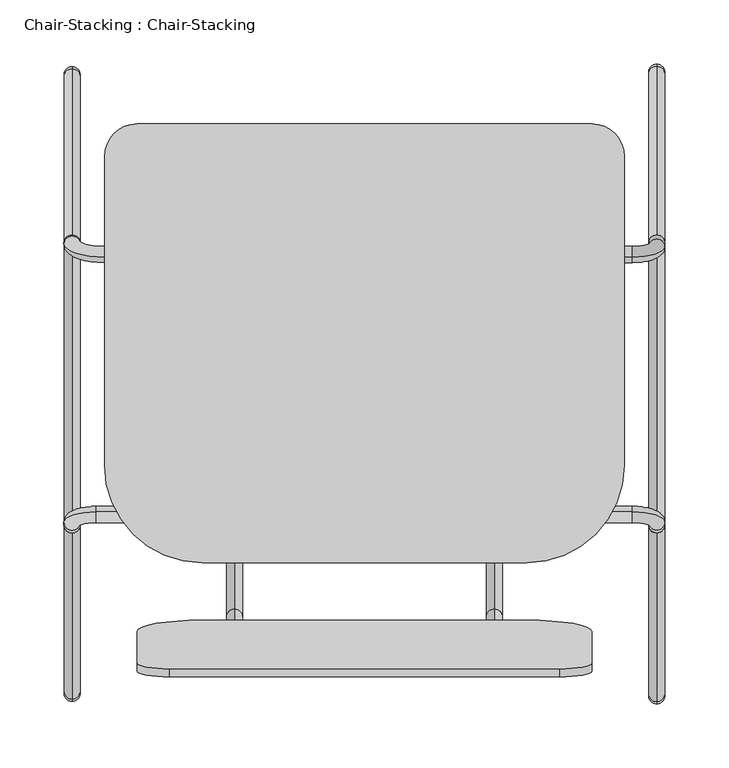
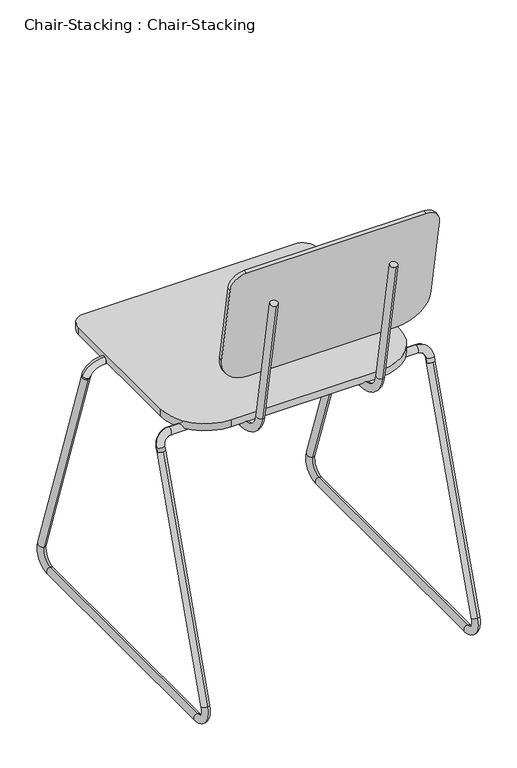
"""IFC4 building model written with IfcOpenShell, lengths in millimetres: furniture geometry, Chair-Stacking : Chair-Stacking."""

from ifc_helpers import new_model, si_unit, point, frame, frame_2d, origin, place, context, project, spatial, polyline, circle_curve, ellipse_curve, trimmed, segment, composite_curve, outline, extrude, source, transform, mapped, element, save
from ifc_brep_helpers import plane_surface, cylinder_surface, revolved_surface, advanced_brep


def chair_stacking_chair_stacking_76f41a28(model_context):
    return source(origin(), model_context, "Body", "SolidModel", [
        advanced_brep(
        [(-280.6491803, 213.2656675, 431.8), (-280.6491803, 213.2656675, 444.5), (-280.6491803, -23.0277124, 431.8), (-280.6491803, -23.0277124, 444.5), (-280.6491803, -66.802417, 481.2313385), (-280.6491803, -79.3094755, 479.0260066), (-280.6491803, -119.2282049, 705.4163709), (-280.6491803, -106.7211464, 707.6217027)],
        [
            (0, 1, circle_curve(frame((-280.6491803, 213.2656675, 438.15), z_axis=(0.0, 1.0, 0.0), x_axis=(0.0, 0.0, 1.0)), 6.35)),
            (1, 0, circle_curve(frame((-280.6491803, 213.2656675, 438.15), z_axis=(0.0, 1.0, 0.0), x_axis=(0.0, 0.0, 1.0)), 6.35)),
            (0, 2),
            (2, 3, circle_curve(frame((-280.6491803, -23.0277124, 438.15), z_axis=(0.0, 1.0, 0.0), x_axis=(0.0, 0.0, 1.0)), 6.35)),
            (3, 1),
            (3, 2, circle_curve(frame((-280.6491803, -23.0277124, 438.15), z_axis=(0.0, 1.0, 0.0), x_axis=(0.0, 0.0, 1.0)), 6.35)),
            (4, 3, circle_curve(frame((-280.6491803, -23.0277124, 488.95), z_axis=(1.0, 0.0, 0.0), x_axis=(0.0, 0.0, -1.0)), 44.45)),
            (2, 5, circle_curve(frame((-280.6491803, -23.0277124, 488.95), z_axis=(-1.0, 0.0, 0.0), x_axis=(0.0, 0.0, -1.0)), 57.15)),
            (5, 4, circle_curve(frame((-280.6491803, -73.0559463, 480.1286726), z_axis=(0.0, 0.17364817766693444, -0.9848077530122074), x_axis=(0.0, 0.9848077530122074, 0.17364817766693444)), 6.35)),
            (4, 5, circle_curve(frame((-280.6491803, -73.0559463, 480.1286726), z_axis=(0.0, 0.17364817766693444, -0.9848077530122074), x_axis=(0.0, 0.9848077530122074, 0.17364817766693444)), 6.35)),
            (6, 7, circle_curve(frame((-280.6491803, -112.9746757, 706.5190368), z_axis=(0.0, -0.1736481776669348, 0.9848077530122074), x_axis=(0.0, 0.9848077530122074, 0.1736481776669348)), 6.35)),
            (7, 6, circle_curve(frame((-280.6491803, -112.9746757, 706.5190368), z_axis=(0.0, -0.1736481776669348, 0.9848077530122074), x_axis=(0.0, 0.9848077530122074, 0.1736481776669348)), 6.35)),
            (5, 6),
            (7, 4),
        ],
        [
            plane_surface(frame((-286.9991803, 213.2656675, 438.15), z_axis=(0.0, 1.0, 0.0), x_axis=(0.0, 0.0, -1.0))),
            cylinder_surface(frame((-280.6491803, 213.2656675, 438.15), z_axis=(0.0, 1.0, 0.0), x_axis=(0.0, 0.0, 1.0)), 6.35),
            revolved_surface(trimmed(ellipse_curve(frame((-280.6491803, -23.0277124, 438.15), z_axis=(0.0, 1.0, 0.0), x_axis=(0.0, 0.0, 1.0)), 6.35, 6.35), [point((-280.6491803, -23.0277124, 431.8))], [point((-280.6491803, -23.0277124, 444.5))], True, "CARTESIAN"), (-280.6491803, -23.0277124, 488.95), (-1.0, 0.0, 0.0)),
            revolved_surface(trimmed(ellipse_curve(frame((-280.6491803, -23.0277124, 438.15), z_axis=(0.0, 1.0, 0.0), x_axis=(0.0, 0.0, 1.0)), 6.35, 6.35), [point((-280.6491803, -23.0277124, 444.5))], [point((-280.6491803, -23.0277124, 431.8))], True, "CARTESIAN"), (-280.6491803, -23.0277124, 488.95), (-1.0, 0.0, 0.0)),
            plane_surface(frame((-280.6491803, -119.2282049, 705.4163709), z_axis=(0.0, -0.17364817766692842, 0.9848077530122085), x_axis=(1.0, 0.0, 0.0))),
            cylinder_surface(frame((-280.6491803, -73.0559463, 480.1286726), z_axis=(0.0, 0.1736481776669348, -0.9848077530122074), x_axis=(0.0, 0.9848077530122074, 0.1736481776669348)), 6.35),
        ],
        [
            (0, [[1, 2]]),
            (1, [[-1, 3, 4, 5]]),
            (1, [[-2, -5, 6, -3]]),
            (2, [[7, -4, 8, 9]]),
            (3, [[-8, -6, -7, 10]]),
            (4, [[11, 12]]),
            (5, [[-9, 13, -12, 14]]),
            (5, [[-10, -14, -11, -13]]),
        ],
    ),
        advanced_brep(
        [(-77.4491803, 213.2656675, 431.8), (-77.4491803, 213.2656675, 444.5), (-77.4491803, -23.0277124, 431.8), (-77.4491803, -23.0277124, 444.5), (-77.4491803, -66.802417, 481.2313385), (-77.4491803, -79.3094755, 479.0260066), (-77.4491803, -118.9339087, 703.7473341), (-77.4491803, -106.4268502, 705.9526659)],
        [
            (0, 1, circle_curve(frame((-77.4491803, 213.2656675, 438.15), z_axis=(0.0, 1.0, 0.0), x_axis=(0.0, 0.0, 1.0)), 6.35)),
            (1, 0, circle_curve(frame((-77.4491803, 213.2656675, 438.15), z_axis=(0.0, 1.0, 0.0), x_axis=(0.0, 0.0, 1.0)), 6.35)),
            (0, 2),
            (2, 3, circle_curve(frame((-77.4491803, -23.0277124, 438.15), z_axis=(0.0, 1.0, 0.0), x_axis=(0.0, 0.0, 1.0)), 6.35)),
            (3, 1),
            (3, 2, circle_curve(frame((-77.4491803, -23.0277124, 438.15), z_axis=(0.0, 1.0, 0.0), x_axis=(0.0, 0.0, 1.0)), 6.35)),
            (4, 3, circle_curve(frame((-77.4491803, -23.0277124, 488.95), z_axis=(1.0, 0.0, 0.0), x_axis=(0.0, 0.0, -1.0)), 44.45)),
            (2, 5, circle_curve(frame((-77.4491803, -23.0277124, 488.95), z_axis=(-1.0, 0.0, 0.0), x_axis=(0.0, 0.0, -1.0)), 57.15)),
            (5, 4, circle_curve(frame((-77.4491803, -73.0559463, 480.1286726), z_axis=(0.0, 0.1736481776669385, -0.9848077530122066), x_axis=(0.0, 0.9848077530122066, 0.1736481776669385)), 6.35)),
            (4, 5, circle_curve(frame((-77.4491803, -73.0559463, 480.1286726), z_axis=(0.0, 0.1736481776669372, -0.9848077530122068), x_axis=(0.0, 0.9848077530122068, 0.1736481776669372)), 6.35)),
            (6, 7, circle_curve(frame((-77.4491803, -112.6803794, 704.85), z_axis=(0.0, -0.17364817766693896, 0.9848077530122066), x_axis=(0.0, 0.9848077530122066, 0.17364817766693896)), 6.35)),
            (7, 6, circle_curve(frame((-77.4491803, -112.6803794, 704.85), z_axis=(0.0, -0.17364817766693896, 0.9848077530122066), x_axis=(0.0, 0.9848077530122066, 0.17364817766693896)), 6.35)),
            (5, 6),
            (7, 4),
        ],
        [
            plane_surface(frame((-83.7991803, 213.2656675, 438.15), z_axis=(0.0, 1.0, 0.0), x_axis=(0.0, 0.0, -1.0))),
            cylinder_surface(frame((-77.4491803, 213.2656675, 438.15), z_axis=(0.0, 1.0, 0.0), x_axis=(0.0, 0.0, 1.0)), 6.35),
            revolved_surface(trimmed(ellipse_curve(frame((-77.4491803, -23.0277124, 438.15), z_axis=(0.0, 1.0, 0.0), x_axis=(0.0, 0.0, 1.0)), 6.35, 6.35), [point((-77.4491803, -23.0277124, 431.8))], [point((-77.4491803, -23.0277124, 444.5))], True, "CARTESIAN"), (-77.4491803, -23.0277124, 488.95), (-1.0, 0.0, 0.0)),
            revolved_surface(trimmed(ellipse_curve(frame((-77.4491803, -23.0277124, 438.15), z_axis=(0.0, 1.0, 0.0), x_axis=(0.0, 0.0, 1.0)), 6.35, 6.35), [point((-77.4491803, -23.0277124, 444.5))], [point((-77.4491803, -23.0277124, 431.8))], True, "CARTESIAN"), (-77.4491803, -23.0277124, 488.95), (-1.0, 0.0, 0.0)),
            plane_surface(frame((-77.4491803, -118.9339087, 703.7473341), z_axis=(0.0, -0.17364817766692892, 0.9848077530122084), x_axis=(1.0, 0.0, 0.0))),
            cylinder_surface(frame((-77.4491803, -73.0559463, 480.1286726), z_axis=(0.0, 0.17364817766693896, -0.9848077530122066), x_axis=(0.0, 0.9848077530122066, 0.17364817766693896)), 6.35),
        ],
        [
            (0, [[1, 2]]),
            (1, [[-1, 3, 4, 5]]),
            (1, [[-2, -5, 6, -3]]),
            (2, [[7, -4, 8, 9]]),
            (3, [[-8, -6, -7, 10]]),
            (4, [[11, 12]]),
            (5, [[-9, 13, -12, 14]]),
            (5, [[-10, -14, -11, -13]]),
        ],
    ),
        extrude(outline(composite_curve([segment(trimmed(circle_curve(frame_2d((-1.2491803, 286.7314636)), 25.4), [point((-1.2491803, 312.1314636))], [point((24.1508197, 286.7314636))], False, "CARTESIAN"), True, "CONTINUOUS"), segment(polyline([(24.1508197, 286.7314636), (24.1508197, 45.4314636)]), True, "CONTINUOUS"), segment(trimmed(circle_curve(frame_2d((-52.0491803, 45.4314636)), 76.2), [point((24.1508197, 45.4314636))], [point((-52.0491803, -30.7685364))], False, "CARTESIAN"), True, "CONTINUOUS"), segment(polyline([(-52.0491803, -30.7685364), (-306.0491803, -30.7685364)]), True, "CONTINUOUS"), segment(trimmed(circle_curve(frame_2d((-306.0491803, 45.4314636)), 76.2), [point((-306.0491803, -30.7685364))], [point((-382.2491803, 45.4314636))], False, "CARTESIAN"), True, "CONTINUOUS"), segment(polyline([(-382.2491803, 45.4314636), (-382.2491803, 286.7314636)]), True, "CONTINUOUS"), segment(trimmed(circle_curve(frame_2d((-356.8491803, 286.7314636)), 25.4), [point((-382.2491803, 286.7314636))], [point((-356.8491803, 312.1314636))], False, "CARTESIAN"), True, "CONTINUOUS"), segment(polyline([(-356.8491803, 312.1314636), (-1.2491803, 312.1314636)]), True, "CONTINUOUS")], self_intersect=False)), frame((0.0, 0.0, 444.5), z_axis=(0.0, 0.0, 1.0), x_axis=(1.0, 0.0, 0.0)), (0.0, 0.0, 1.0), 12.7),
        extrude(outline(composite_curve([segment(polyline([(-304.8, 0.0), (0.0, 0.0)]), True, "CONTINUOUS"), segment(trimmed(circle_curve(frame_2d((0.0, -25.4)), 25.4), [point((0.0, 0.0))], [point((25.4, -25.4))], False, "CARTESIAN"), True, "CONTINUOUS"), segment(polyline([(25.4, -25.4), (25.4, -168.3013626)]), True, "CONTINUOUS"), segment(trimmed(circle_curve(frame_2d((-25.4, -168.3013626)), 50.8), [point((25.4, -168.3013626))], [point((-25.4, -219.1013626))], False, "CARTESIAN"), True, "CONTINUOUS"), segment(polyline([(-25.4, -219.1013626), (-279.4, -219.1013626)]), True, "CONTINUOUS"), segment(trimmed(circle_curve(frame_2d((-279.4, -168.3013626)), 50.8), [point((-279.4, -219.1013626))], [point((-330.2, -168.3013626))], False, "CARTESIAN"), True, "CONTINUOUS"), segment(polyline([(-330.2, -168.3013626), (-330.2, -25.4)]), True, "CONTINUOUS"), segment(trimmed(circle_curve(frame_2d((-304.8, -25.4)), 25.4), [point((-330.2, -25.4))], [point((-304.8, 0.0))], False, "CARTESIAN"), True, "CONTINUOUS")], self_intersect=False)), frame((-331.4491803, -119.9531376, 782.6640535), z_axis=(0.0, 0.9848077530122084, 0.17364817766692858), x_axis=(-1.0, 0.0, 0.0)), (0.0, 0.0, 1.0), 6.35),
        advanced_brep(
        [(55.9008197, 219.2327758, 419.1211728), (43.2008197, 219.2327758, 419.1211728), (55.9008197, 216.3017292, 427.6700586), (43.2008197, 216.3017292, 427.6700586), (30.5008197, 212.1828103, 439.6835721), (30.5008197, 208.0638914, 451.6970857), (-382.2491803, 208.0638914, 451.6970857), (-382.2491803, 212.1828103, 439.6835721), (-401.2991803, 218.3611887, 421.6633019), (-413.9991803, 218.3611887, 421.6633019), (-413.9991803, 219.2424531, 419.0929473), (-401.2991803, 219.2424531, 419.0929473)],
        [
            (0, 1, circle_curve(frame((49.5508197, 219.2327758, 419.1211728), z_axis=(0.0, 0.32432432432432967, -0.9459459459459442), x_axis=(-1.0, 0.0, 0.0)), 6.35)),
            (1, 0, circle_curve(frame((49.5508197, 219.2327758, 419.1211728), z_axis=(0.0, 0.32432432432432967, -0.9459459459459442), x_axis=(-1.0, 0.0, 0.0)), 6.35)),
            (0, 2),
            (2, 3, circle_curve(frame((49.5508197, 216.3017292, 427.6700586), z_axis=(0.0, 0.32432432432432967, -0.9459459459459442), x_axis=(-1.0, 0.0, 0.0)), 6.35)),
            (3, 1),
            (3, 2, circle_curve(frame((49.5508197, 216.3017292, 427.6700586), z_axis=(0.0, 0.32432432432432967, -0.9459459459459442), x_axis=(-1.0, 0.0, 0.0)), 6.35)),
            (4, 3, circle_curve(frame((30.5008197, 216.3017292, 427.6700586), z_axis=(0.0, 0.9459459459459447, 0.3243243243243281), x_axis=(1.0, 0.0, 0.0)), 12.7)),
            (2, 5, circle_curve(frame((30.5008197, 216.3017292, 427.6700586), z_axis=(0.0, -0.9459459459459447, -0.3243243243243281), x_axis=(1.0, 0.0, 0.0)), 25.4)),
            (5, 4, circle_curve(frame((30.5008197, 210.1233509, 445.6903289), z_axis=(1.0, 0.0, 0.0), x_axis=(0.0, 0.32432432432432745, -0.9459459459459449)), 6.35)),
            (4, 5, circle_curve(frame((30.5008197, 210.1233509, 445.6903289), z_axis=(1.0, 0.0, 0.0), x_axis=(0.0, 0.32432432432432745, -0.9459459459459449)), 6.35)),
            (5, 6),
            (6, 7, circle_curve(frame((-382.2491803, 210.1233509, 445.6903289), z_axis=(1.0, 0.0, 0.0), x_axis=(0.0, 0.32432432432432745, -0.9459459459459449)), 6.35)),
            (7, 4),
            (7, 6, circle_curve(frame((-382.2491803, 210.1233509, 445.6903289), z_axis=(1.0, 0.0, 0.0), x_axis=(0.0, 0.32432432432432745, -0.9459459459459449)), 6.35)),
            (8, 7, circle_curve(frame((-382.2491803, 218.3611887, 421.6633019), z_axis=(0.0, 0.9459459459459447, 0.3243243243243281), x_axis=(0.0, -0.3243243243243281, 0.9459459459459447)), 19.05)),
            (6, 9, circle_curve(frame((-382.2491803, 218.3611887, 421.6633019), z_axis=(0.0, -0.9459459459459447, -0.3243243243243281), x_axis=(0.0, -0.3243243243243281, 0.9459459459459447)), 31.75)),
            (9, 8, circle_curve(frame((-407.6491803, 218.3611887, 421.6633019), z_axis=(0.0, -0.324324324324328, 0.9459459459459447), x_axis=(1.0000000000000002, 0.0, 0.0)), 6.35)),
            (8, 9, circle_curve(frame((-407.6491803, 218.3611887, 421.6633019), z_axis=(0.0, -0.324324324324328, 0.9459459459459447), x_axis=(1.0000000000000002, 0.0, 0.0)), 6.35)),
            (10, 11, circle_curve(frame((-407.6491803, 219.2424531, 419.0929473), z_axis=(0.0, 0.32432432432432784, -0.9459459459459449), x_axis=(1.0, 0.0, 0.0)), 6.35)),
            (11, 10, circle_curve(frame((-407.6491803, 219.2424531, 419.0929473), z_axis=(0.0, 0.32432432432432784, -0.9459459459459449), x_axis=(1.0, 0.0, 0.0)), 6.35)),
            (9, 10),
            (11, 8),
        ],
        [
            plane_surface(frame((49.5508197, 213.226019, 417.0617133), z_axis=(0.0, 0.32432432432433117, -0.9459459459459437), x_axis=(1.0, 0.0, 0.0))),
            cylinder_surface(frame((49.5508197, 219.2327758, 419.1211728), z_axis=(0.0, 0.32432432432432967, -0.9459459459459442), x_axis=(-1.0, 0.0, 0.0)), 6.35),
            revolved_surface(trimmed(ellipse_curve(frame((49.5508197, 216.3017292, 427.6700586), z_axis=(0.0, 0.32432432432432823, -0.9459459459459447), x_axis=(-1.0, 0.0, 0.0)), 6.35, 6.35), [point((55.9008197, 216.3017292, 427.6700586))], [point((43.2008197, 216.3017292, 427.6700586))], True, "CARTESIAN"), (30.5008197, 216.3017292, 427.6700586), (0.0, -0.9459459459459447, -0.3243243243243281)),
            revolved_surface(trimmed(ellipse_curve(frame((49.5508197, 216.3017292, 427.6700586), z_axis=(0.0, 0.32432432432432823, -0.9459459459459447), x_axis=(-1.0, 0.0, 0.0)), 6.35, 6.35), [point((43.2008197, 216.3017292, 427.6700586))], [point((55.9008197, 216.3017292, 427.6700586))], True, "CARTESIAN"), (30.5008197, 216.3017292, 427.6700586), (0.0, -0.9459459459459447, -0.3243243243243281)),
            cylinder_surface(frame((30.5008197, 210.1233509, 445.6903289), z_axis=(1.0, 0.0, 0.0), x_axis=(0.0, 0.32432432432432745, -0.9459459459459449)), 6.35),
            revolved_surface(trimmed(ellipse_curve(frame((-382.2491803, 210.1233509, 445.6903289), z_axis=(1.0000000000000002, 0.0, 0.0), x_axis=(0.0, 0.3243243243243276, -0.9459459459459448)), 6.35, 6.35), [point((-382.2491803, 208.0638914, 451.6970857))], [point((-382.2491803, 212.1828103, 439.6835721))], True, "CARTESIAN"), (-382.2491803, 218.3611887, 421.6633019), (0.0, -0.9459459459459447, -0.3243243243243281)),
            revolved_surface(trimmed(ellipse_curve(frame((-382.2491803, 210.1233509, 445.6903289), z_axis=(1.0000000000000002, 0.0, 0.0), x_axis=(0.0, 0.3243243243243276, -0.9459459459459448)), 6.35, 6.35), [point((-382.2491803, 212.1828103, 439.6835721))], [point((-382.2491803, 208.0638914, 451.6970857))], True, "CARTESIAN"), (-382.2491803, 218.3611887, 421.6633019), (0.0, -0.9459459459459447, -0.3243243243243281)),
            plane_surface(frame((-407.6491803, 225.2492099, 421.1524068), z_axis=(0.0, 0.3243243243243264, -0.9459459459459453), x_axis=(1.0, 0.0, 0.0))),
            cylinder_surface(frame((-407.6491803, 218.3611887, 421.6633019), z_axis=(0.0, -0.3243243243243278, 0.9459459459459447), x_axis=(1.0, 0.0, 0.0)), 6.35),
        ],
        [
            (0, [[1, 2]]),
            (1, [[-1, 3, 4, 5]]),
            (1, [[-2, -5, 6, -3]]),
            (2, [[7, -4, 8, 9]]),
            (3, [[-8, -6, -7, 10]]),
            (4, [[-9, 11, 12, 13]]),
            (4, [[-10, -13, 14, -11]]),
            (5, [[15, -12, 16, 17]]),
            (6, [[-16, -14, -15, 18]]),
            (7, [[19, 20]]),
            (8, [[-17, 21, -20, 22]]),
            (8, [[-18, -22, -19, -21]]),
        ],
    ),
        advanced_brep(
        [(55.9008197, -1.3812406, 419.0879461), (43.2008197, -1.3812406, 419.0879461), (55.9008197, 0.7944914, 425.4338312), (43.2008197, 0.7944914, 425.4338312), (30.5008197, 4.9134104, 437.4473447), (30.5008197, 9.0323293, 449.4608582), (-388.5991803, 9.0323293, 449.4608582), (-388.5991803, 4.9134104, 437.4473447), (-401.2991803, 0.7944914, 425.4338312), (-413.9991803, 0.7944914, 425.4338312), (-413.9991803, -1.3997864, 419.0338542), (-401.2991803, -1.3997864, 419.0338542)],
        [
            (0, 1, circle_curve(frame((49.5508197, -1.3812406, 419.0879461), z_axis=(0.0, -0.32432432432432495, -0.9459459459459457), x_axis=(-1.0, 0.0, 0.0)), 6.35)),
            (1, 0, circle_curve(frame((49.5508197, -1.3812406, 419.0879461), z_axis=(0.0, -0.32432432432432495, -0.9459459459459457), x_axis=(-1.0, 0.0, 0.0)), 6.35)),
            (0, 2),
            (2, 3, circle_curve(frame((49.5508197, 0.7944914, 425.4338312), z_axis=(0.0, -0.32432432432432495, -0.9459459459459457), x_axis=(-1.0, 0.0, 0.0)), 6.35)),
            (3, 1),
            (3, 2, circle_curve(frame((49.5508197, 0.7944914, 425.4338312), z_axis=(0.0, -0.32432432432432495, -0.9459459459459457), x_axis=(-1.0, 0.0, 0.0)), 6.35)),
            (4, 3, circle_curve(frame((30.5008197, 0.7944914, 425.4338312), z_axis=(0.0, 0.9459459459459458, -0.3243243243243246), x_axis=(1.0, 0.0, 0.0)), 12.7)),
            (2, 5, circle_curve(frame((30.5008197, 0.7944914, 425.4338312), z_axis=(0.0, -0.9459459459459458, 0.3243243243243246), x_axis=(1.0, 0.0, 0.0)), 25.4)),
            (5, 4, circle_curve(frame((30.5008197, 6.9728698, 443.4541014), z_axis=(1.0, 0.0, 0.0), x_axis=(0.0, -0.3243243243243236, -0.9459459459459462)), 6.35)),
            (4, 5, circle_curve(frame((30.5008197, 6.9728698, 443.4541014), z_axis=(1.0, 0.0, 0.0), x_axis=(0.0, -0.3243243243243236, -0.9459459459459462)), 6.35)),
            (5, 6),
            (6, 7, circle_curve(frame((-388.5991803, 6.9728698, 443.4541014), z_axis=(1.0, 0.0, 0.0), x_axis=(0.0, -0.3243243243243236, -0.9459459459459462)), 6.35)),
            (7, 4),
            (7, 6, circle_curve(frame((-388.5991803, 6.9728698, 443.4541014), z_axis=(1.0, 0.0, 0.0), x_axis=(0.0, -0.3243243243243236, -0.9459459459459462)), 6.35)),
            (8, 7, circle_curve(frame((-388.5991803, 0.7944914, 425.4338312), z_axis=(0.0, 0.9459459459459458, -0.3243243243243246), x_axis=(0.0, 0.3243243243243246, 0.9459459459459458)), 12.7)),
            (6, 9, circle_curve(frame((-388.5991803, 0.7944914, 425.4338312), z_axis=(0.0, -0.9459459459459458, 0.3243243243243246), x_axis=(0.0, 0.3243243243243246, 0.9459459459459458)), 25.4)),
            (9, 8, circle_curve(frame((-407.6491803, 0.7944914, 425.4338312), z_axis=(0.0, 0.3243243243243247, 0.9459459459459458), x_axis=(1.0, 0.0, 0.0)), 6.35)),
            (8, 9, circle_curve(frame((-407.6491803, 0.7944914, 425.4338312), z_axis=(0.0, 0.3243243243243247, 0.9459459459459458), x_axis=(1.0, 0.0, 0.0)), 6.35)),
            (10, 11, circle_curve(frame((-407.6491803, -1.3997864, 419.0338542), z_axis=(0.0, -0.3243243243243242, -0.945945945945946), x_axis=(1.0, 0.0, 0.0)), 6.35)),
            (11, 10, circle_curve(frame((-407.6491803, -1.3997864, 419.0338542), z_axis=(0.0, -0.3243243243243242, -0.945945945945946), x_axis=(1.0, 0.0, 0.0)), 6.35)),
            (9, 10),
            (11, 8),
        ],
        [
            plane_surface(frame((49.5508197, -7.3879973, 421.1474055), z_axis=(0.0, -0.32432432432432273, -0.9459459459459466), x_axis=(1.0, 0.0, 0.0))),
            cylinder_surface(frame((49.5508197, -1.3812406, 419.0879461), z_axis=(0.0, -0.32432432432432495, -0.9459459459459457), x_axis=(-1.0, 0.0, 0.0)), 6.35),
            revolved_surface(trimmed(ellipse_curve(frame((49.5508197, 0.7944914, 425.4338312), z_axis=(0.0, -0.32432432432432456, -0.9459459459459458), x_axis=(-1.0, 0.0, 0.0)), 6.35, 6.35), [point((55.9008197, 0.7944914, 425.4338312))], [point((43.2008197, 0.7944914, 425.4338312))], True, "CARTESIAN"), (30.5008197, 0.7944914, 425.4338312), (0.0, -0.9459459459459458, 0.3243243243243246)),
            revolved_surface(trimmed(ellipse_curve(frame((49.5508197, 0.7944914, 425.4338312), z_axis=(0.0, -0.32432432432432456, -0.9459459459459458), x_axis=(-1.0, 0.0, 0.0)), 6.35, 6.35), [point((43.2008197, 0.7944914, 425.4338312))], [point((55.9008197, 0.7944914, 425.4338312))], True, "CARTESIAN"), (30.5008197, 0.7944914, 425.4338312), (0.0, -0.9459459459459458, 0.3243243243243246)),
            cylinder_surface(frame((30.5008197, 6.9728698, 443.4541014), z_axis=(1.0, 0.0, 0.0), x_axis=(0.0, -0.3243243243243236, -0.9459459459459462)), 6.35),
            revolved_surface(trimmed(ellipse_curve(frame((-388.5991803, 6.9728698, 443.4541014), z_axis=(1.0, 0.0, 0.0), x_axis=(0.0, -0.3243243243243236, -0.9459459459459462)), 6.35, 6.35), [point((-388.5991803, 9.0323293, 449.4608582))], [point((-388.5991803, 4.9134104, 437.4473447))], True, "CARTESIAN"), (-388.5991803, 0.7944914, 425.4338312), (0.0, -0.9459459459459458, 0.3243243243243246)),
            revolved_surface(trimmed(ellipse_curve(frame((-388.5991803, 6.9728698, 443.4541014), z_axis=(1.0, 0.0, 0.0), x_axis=(0.0, -0.3243243243243236, -0.9459459459459462)), 6.35, 6.35), [point((-388.5991803, 4.9134104, 437.4473447))], [point((-388.5991803, 9.0323293, 449.4608582))], True, "CARTESIAN"), (-388.5991803, 0.7944914, 425.4338312), (0.0, -0.9459459459459458, 0.3243243243243246)),
            plane_surface(frame((-407.6491803, 4.6069704, 416.9743947), z_axis=(0.0, -0.3243243243243226, -0.9459459459459466), x_axis=(1.0, 0.0, 0.0))),
            cylinder_surface(frame((-407.6491803, 0.7944914, 425.4338312), z_axis=(0.0, 0.3243243243243242, 0.945945945945946), x_axis=(1.0, 0.0, 0.0)), 6.35),
        ],
        [
            (0, [[1, 2]]),
            (1, [[-1, 3, 4, 5]]),
            (1, [[-2, -5, 6, -3]]),
            (2, [[7, -4, 8, 9]]),
            (3, [[-8, -6, -7, 10]]),
            (4, [[-9, 11, 12, 13]]),
            (4, [[-10, -13, 14, -11]]),
            (5, [[15, -12, 16, 17]]),
            (6, [[-16, -14, -15, 18]]),
            (7, [[19, 20]]),
            (8, [[-17, 21, -20, 22]]),
            (8, [[-18, -22, -19, -21]]),
        ],
    ),
        advanced_brep(
        [(-407.6491803, 225.2492099, 421.1524068), (-407.6491803, 213.2356963, 417.0334879), (-407.6491803, 355.2281045, 42.0472973), (-407.6491803, 343.214591, 37.9283784), (-407.6491803, 325.1943208, 12.7), (-407.6491803, 325.1943208, 0.0), (-407.6491803, -107.3313935, 0.0), (-407.6491803, -107.3313935, 12.7), (-407.6491803, -125.3516638, 37.9283784), (-407.6491803, -137.3651773, 42.0472973), (-407.6491803, -7.4065431, 421.0933136), (-407.6491803, 4.6069704, 416.9743947)],
        [
            (0, 1, circle_curve(frame((-407.6491803, 219.2424531, 419.0929473), z_axis=(0.0, -0.3243243243243311, 0.9459459459459437), x_axis=(0.0, -0.9459459459459437, -0.3243243243243311)), 6.35)),
            (1, 0, circle_curve(frame((-407.6491803, 219.2424531, 419.0929473), z_axis=(0.0, -0.3243243243243311, 0.9459459459459437), x_axis=(0.0, -0.9459459459459437, -0.3243243243243311)), 6.35)),
            (0, 2),
            (2, 3, circle_curve(frame((-407.6491803, 349.2213478, 39.9878378), z_axis=(0.0, -0.3243243243243311, 0.9459459459459437), x_axis=(0.0, -0.9459459459459437, -0.3243243243243311)), 6.35)),
            (3, 1),
            (3, 2, circle_curve(frame((-407.6491803, 349.2213478, 39.9878378), z_axis=(0.0, -0.3243243243243311, 0.9459459459459437), x_axis=(0.0, -0.9459459459459437, -0.3243243243243311)), 6.35)),
            (4, 3, circle_curve(frame((-407.6491803, 325.1943208, 31.75), z_axis=(1.0, 0.0, 0.0), x_axis=(0.0, 0.9459459459459434, 0.3243243243243317)), 19.05)),
            (2, 5, circle_curve(frame((-407.6491803, 325.1943208, 31.75), z_axis=(-1.0, 0.0, 0.0), x_axis=(0.0, 0.9459459459459434, 0.3243243243243317)), 31.75)),
            (5, 4, circle_curve(frame((-407.6491803, 325.1943208, 6.35), z_axis=(0.0, 1.0, 0.0), x_axis=(0.0, 0.0, 1.0)), 6.35)),
            (4, 5, circle_curve(frame((-407.6491803, 325.1943208, 6.35), z_axis=(0.0, 0.9999999999999999, 0.0), x_axis=(0.0, 0.0, 0.9999999999999999)), 6.35)),
            (5, 6),
            (6, 7, circle_curve(frame((-407.6491803, -107.3313935, 6.35), z_axis=(0.0, 1.0, 0.0), x_axis=(0.0, 0.0, 1.0)), 6.35)),
            (7, 4),
            (7, 6, circle_curve(frame((-407.6491803, -107.3313935, 6.35), z_axis=(0.0, 1.0, 0.0), x_axis=(0.0, 0.0, 1.0)), 6.35)),
            (8, 7, circle_curve(frame((-407.6491803, -107.3313935, 31.75), z_axis=(1.0, 0.0, 0.0), x_axis=(0.0, 0.0, -1.0)), 19.05)),
            (6, 9, circle_curve(frame((-407.6491803, -107.3313935, 31.75), z_axis=(-1.0, 0.0, 0.0), x_axis=(0.0, 0.0, -1.0)), 31.75)),
            (9, 8, circle_curve(frame((-407.6491803, -131.3584206, 39.9878378), z_axis=(0.0, -0.3243243243243189, -0.9459459459459478), x_axis=(0.0, 0.9459459459459478, -0.3243243243243189)), 6.35)),
            (8, 9, circle_curve(frame((-407.6491803, -131.3584206, 39.9878378), z_axis=(0.0, -0.3243243243243206, -0.9459459459459473), x_axis=(0.0, 0.9459459459459473, -0.3243243243243206)), 6.35)),
            (10, 11, circle_curve(frame((-407.6491803, -1.3997864, 419.0338542), z_axis=(0.0, 0.3243243243243217, 0.9459459459459468), x_axis=(0.0, 0.9459459459459468, -0.3243243243243217)), 6.35)),
            (11, 10, circle_curve(frame((-407.6491803, -1.3997864, 419.0338542), z_axis=(0.0, 0.3243243243243217, 0.9459459459459468), x_axis=(0.0, 0.9459459459459468, -0.3243243243243217)), 6.35)),
            (9, 10),
            (11, 8),
        ],
        [
            plane_surface(frame((-407.6491803, 225.2492099, 421.1524068), z_axis=(0.0, -0.32432432432432773, 0.9459459459459448), x_axis=(1.0, 0.0, 0.0))),
            cylinder_surface(frame((-407.6491803, 219.2424531, 419.0929473), z_axis=(0.0, -0.3243243243243311, 0.9459459459459437), x_axis=(0.0, -0.9459459459459437, -0.3243243243243311)), 6.35),
            revolved_surface(trimmed(ellipse_curve(frame((-407.6491803, 349.2213478, 39.9878378), z_axis=(0.0, -0.3243243243243347, 0.9459459459459424), x_axis=(0.0, -0.9459459459459424, -0.3243243243243347)), 6.35, 6.35), [point((-407.6491803, 355.2281045, 42.0472973))], [point((-407.6491803, 343.214591, 37.9283784))], True, "CARTESIAN"), (-407.6491803, 325.1943208, 31.75), (-1.0, 0.0, 0.0)),
            revolved_surface(trimmed(ellipse_curve(frame((-407.6491803, 349.2213478, 39.9878378), z_axis=(0.0, -0.3243243243243347, 0.9459459459459424), x_axis=(0.0, -0.9459459459459424, -0.3243243243243347)), 6.35, 6.35), [point((-407.6491803, 343.214591, 37.9283784))], [point((-407.6491803, 355.2281045, 42.0472973))], True, "CARTESIAN"), (-407.6491803, 325.1943208, 31.75), (-1.0, 0.0, 0.0)),
            cylinder_surface(frame((-407.6491803, 325.1943208, 6.35), z_axis=(0.0, 1.0, 0.0), x_axis=(0.0, 0.0, 1.0)), 6.35),
            revolved_surface(trimmed(ellipse_curve(frame((-407.6491803, -107.3313935, 6.35), z_axis=(0.0, 1.0, 0.0), x_axis=(0.0, 0.0, 1.0)), 6.35, 6.35), [point((-407.6491803, -107.3313935, 0.0))], [point((-407.6491803, -107.3313935, 12.7))], True, "CARTESIAN"), (-407.6491803, -107.3313935, 31.75), (-1.0, 0.0, 0.0)),
            revolved_surface(trimmed(ellipse_curve(frame((-407.6491803, -107.3313935, 6.35), z_axis=(0.0, 1.0, 0.0), x_axis=(0.0, 0.0, 1.0)), 6.35, 6.35), [point((-407.6491803, -107.3313935, 12.7))], [point((-407.6491803, -107.3313935, 0.0))], True, "CARTESIAN"), (-407.6491803, -107.3313935, 31.75), (-1.0, 0.0, 0.0)),
            plane_surface(frame((-407.6491803, -7.4065431, 421.0933136), z_axis=(0.0, 0.324324324324323, 0.9459459459459465), x_axis=(1.0, 0.0, 0.0))),
            cylinder_surface(frame((-407.6491803, -131.3584206, 39.9878378), z_axis=(0.0, -0.3243243243243217, -0.9459459459459468), x_axis=(0.0, 0.9459459459459468, -0.3243243243243217)), 6.35),
        ],
        [
            (0, [[1, 2]]),
            (1, [[-1, 3, 4, 5]]),
            (1, [[-2, -5, 6, -3]]),
            (2, [[7, -4, 8, 9]]),
            (3, [[-8, -6, -7, 10]]),
            (4, [[-9, 11, 12, 13]]),
            (4, [[-10, -13, 14, -11]]),
            (5, [[15, -12, 16, 17]]),
            (6, [[-16, -14, -15, 18]]),
            (7, [[19, 20]]),
            (8, [[-17, 21, -20, 22]]),
            (8, [[-18, -22, -19, -21]]),
        ],
    ),
        advanced_brep(
        [(49.5508197, 225.2597598, 421.1875673), (49.5508197, 213.2656675, 417.0124327), (49.5508197, 357.1892841, 42.1878365), (49.5508197, 345.1951918, 38.0127019), (49.5508197, 327.2040533, 12.7), (49.5508197, 327.2040533, 0.0), (49.5508197, -109.3411268, 0.0), (49.5508197, -109.3411268, 12.7), (49.5508197, -127.3337908, 38.0083179), (49.5508197, -139.3289001, 42.1805298), (49.5508197, -7.5008737, 421.186106), (49.5508197, 4.4942357, 417.013894)],
        [
            (0, 1, circle_curve(frame((49.5508197, 219.2627136, 419.1), z_axis=(0.0, -0.3287507573582007, 0.9444167192168982), x_axis=(0.0, -0.9444167192168982, -0.3287507573582007)), 6.35)),
            (1, 0, circle_curve(frame((49.5508197, 219.2627136, 419.1), z_axis=(0.0, -0.3287507573582007, 0.9444167192168982), x_axis=(0.0, -0.9444167192168982, -0.3287507573582007)), 6.35)),
            (0, 2),
            (2, 3, circle_curve(frame((49.5508197, 351.1922379, 40.1002692), z_axis=(0.0, -0.3287507573582007, 0.9444167192168982), x_axis=(0.0, -0.9444167192168982, -0.3287507573582007)), 6.35)),
            (3, 1),
            (3, 2, circle_curve(frame((49.5508197, 351.1922379, 40.1002692), z_axis=(0.0, -0.3287507573582007, 0.9444167192168982), x_axis=(0.0, -0.9444167192168982, -0.3287507573582007)), 6.35)),
            (4, 3, circle_curve(frame((49.5508197, 327.2040533, 31.75), z_axis=(1.0, 0.0, 0.0), x_axis=(0.0, 0.944416719216897, 0.3287507573582041)), 19.05)),
            (2, 5, circle_curve(frame((49.5508197, 327.2040533, 31.75), z_axis=(-1.0, 0.0, 0.0), x_axis=(0.0, 0.944416719216897, 0.3287507573582041)), 31.75)),
            (5, 4, circle_curve(frame((49.5508197, 327.2040533, 6.35), z_axis=(0.0, 1.0, 0.0), x_axis=(0.0, 0.0, 1.0)), 6.35)),
            (4, 5, circle_curve(frame((49.5508197, 327.2040533, 6.35), z_axis=(0.0, 0.9999999999999999, 0.0), x_axis=(0.0, 0.0, 0.9999999999999999)), 6.35)),
            (5, 6),
            (6, 7, circle_curve(frame((49.5508197, -109.3411268, 6.35), z_axis=(0.0, 1.0, 0.0), x_axis=(0.0, 0.0, 1.0)), 6.35)),
            (7, 4),
            (7, 6, circle_curve(frame((49.5508197, -109.3411268, 6.35), z_axis=(0.0, 1.0, 0.0), x_axis=(0.0, 0.0, 1.0)), 6.35)),
            (8, 7, circle_curve(frame((49.5508197, -109.3411268, 31.75), z_axis=(1.0, 0.0, 0.0), x_axis=(0.0, 0.0, -1.0)), 19.05)),
            (6, 9, circle_curve(frame((49.5508197, -109.3411268, 31.75), z_axis=(-1.0, 0.0, 0.0), x_axis=(0.0, 0.0, -1.0)), 31.75)),
            (9, 8, circle_curve(frame((49.5508197, -133.3313455, 40.0944239), z_axis=(0.0, -0.3285206249412718, -0.9444967967061594), x_axis=(0.0, 0.9444967967061594, -0.3285206249412718)), 6.35)),
            (8, 9, circle_curve(frame((49.5508197, -133.3313455, 40.0944239), z_axis=(0.0, -0.3285206249412754, -0.9444967967061582), x_axis=(0.0, 0.9444967967061582, -0.3285206249412754)), 6.35)),
            (10, 11, circle_curve(frame((49.5508197, -1.503319, 419.1), z_axis=(0.0, 0.3285206249412728, 0.9444967967061592), x_axis=(0.0, 0.9444967967061592, -0.3285206249412728)), 6.35)),
            (11, 10, circle_curve(frame((49.5508197, -1.503319, 419.1), z_axis=(0.0, 0.3285206249412728, 0.9444967967061592), x_axis=(0.0, 0.9444967967061592, -0.3285206249412728)), 6.35)),
            (9, 10),
            (11, 8),
        ],
        [
            plane_surface(frame((49.5508197, 225.2597598, 421.1875673), z_axis=(0.0, -0.3287507573582023, 0.9444167192168977), x_axis=(1.0, 0.0, 0.0))),
            cylinder_surface(frame((49.5508197, 219.2627136, 419.1), z_axis=(0.0, -0.3287507573582007, 0.9444167192168982), x_axis=(0.0, -0.9444167192168982, -0.3287507573582007)), 6.35),
            revolved_surface(trimmed(ellipse_curve(frame((49.5508197, 351.1922379, 40.1002692), z_axis=(0.0, -0.32875075735820414, 0.944416719216897), x_axis=(0.0, -0.944416719216897, -0.32875075735820414)), 6.35, 6.35), [point((49.5508197, 357.1892841, 42.1878365))], [point((49.5508197, 345.1951918, 38.0127019))], True, "CARTESIAN"), (49.5508197, 327.2040533, 31.75), (-1.0, 0.0, 0.0)),
            revolved_surface(trimmed(ellipse_curve(frame((49.5508197, 351.1922379, 40.1002692), z_axis=(0.0, -0.32875075735820414, 0.944416719216897), x_axis=(0.0, -0.944416719216897, -0.32875075735820414)), 6.35, 6.35), [point((49.5508197, 345.1951918, 38.0127019))], [point((49.5508197, 357.1892841, 42.1878365))], True, "CARTESIAN"), (49.5508197, 327.2040533, 31.75), (-1.0, 0.0, 0.0)),
            cylinder_surface(frame((49.5508197, 327.2040533, 6.35), z_axis=(0.0, 1.0, 0.0), x_axis=(0.0, 0.0, 1.0)), 6.35),
            revolved_surface(trimmed(ellipse_curve(frame((49.5508197, -109.3411268, 6.35), z_axis=(0.0, 1.0, 0.0), x_axis=(0.0, 0.0, 1.0)), 6.35, 6.35), [point((49.5508197, -109.3411268, 0.0))], [point((49.5508197, -109.3411268, 12.7))], True, "CARTESIAN"), (49.5508197, -109.3411268, 31.75), (-1.0, 0.0, 0.0)),
            revolved_surface(trimmed(ellipse_curve(frame((49.5508197, -109.3411268, 6.35), z_axis=(0.0, 1.0, 0.0), x_axis=(0.0, 0.0, 1.0)), 6.35, 6.35), [point((49.5508197, -109.3411268, 12.7))], [point((49.5508197, -109.3411268, 0.0))], True, "CARTESIAN"), (49.5508197, -109.3411268, 31.75), (-1.0, 0.0, 0.0)),
            plane_surface(frame((49.5508197, -7.5008737, 421.186106), z_axis=(0.0, 0.3285206249412714, 0.9444967967061596), x_axis=(1.0, 0.0, 0.0))),
            cylinder_surface(frame((49.5508197, -133.3313455, 40.0944239), z_axis=(0.0, -0.3285206249412728, -0.9444967967061592), x_axis=(0.0, 0.9444967967061592, -0.3285206249412728)), 6.35),
        ],
        [
            (0, [[1, 2]]),
            (1, [[-1, 3, 4, 5]]),
            (1, [[-2, -5, 6, -3]]),
            (2, [[7, -4, 8, 9]]),
            (3, [[-8, -6, -7, 10]]),
            (4, [[-9, 11, 12, 13]]),
            (4, [[-10, -13, 14, -11]]),
            (5, [[15, -12, 16, 17]]),
            (6, [[-16, -14, -15, 18]]),
            (7, [[19, 20]]),
            (8, [[-17, 21, -20, 22]]),
            (8, [[-18, -22, -19, -21]]),
        ],
    ),
    ])


if __name__ == "__main__":
    model = new_model("IFC4")
    model_context = context("Model", 3, world=origin())
    ifc_project = project(units=[si_unit("LENGTHUNIT", "METRE", prefix="MILLI")], contexts=[model_context])
    site = spatial("IfcSite", under=ifc_project)
    building = spatial("IfcBuilding", under=site)
    placement = place(None, origin())
    chair_stacking_chair_stacking_shape = chair_stacking_chair_stacking_76f41a28(model_context)
    element("IfcFurniture", 1, ObjectType="Chair-Stacking : Chair-Stacking", at=placement, inside=building, context=model_context, shape_type="MappedRepresentation", body=[
        mapped(chair_stacking_chair_stacking_shape, transform((0.0, 0.0, 0.0), x_axis=(1.0, 0.0, 0.0), y_axis=(0.0, 1.0, 0.0), z_axis=(0.0, 0.0, 1.0))),
    ])
    save(model, "model.ifc")

# Revit data of these elements
# Type "Chair-Stacking : Chair-Stacking"
#   Assembly Code = "E2020200"
#   Seat/Back Material = Cherry
#   Default Elevation = 0
# Element 1 (IfcFurniture, "Chair-Stacking : Chair-Stacking")
#   Materials on its faces: "Steel, Chrome Plated", "Cherry"
# Materials
#   "Cherry": class "Wood", colour RGB 226 177 128, transparency 0, Description = "Prunus Serotina", Cost = 0
#   "Steel, Chrome Plated": class "Metal", colour RGB 17 17 17, transparency 0, Description = "Chromiuim plated steel", Cost = 0
